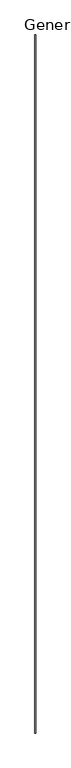
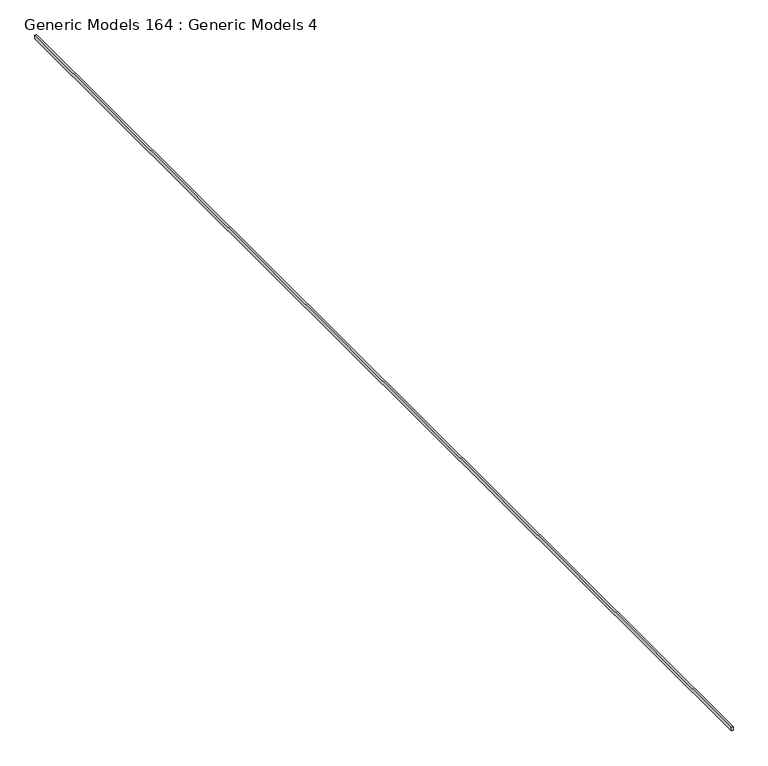
"""IFC4 building model written with IfcOpenShell, lengths in millimetres: proxy geometry, Generic Models 164 : Generic Models 4."""

from ifc_helpers import new_model, si_unit, origin, place, context, project, spatial, faceted_brep, source, transform, mapped, element, save


def generic_models_164_generic_models_4_ca790fd0(model_context):
    return source(origin(), model_context, "Body", "Brep", [
        faceted_brep([(-10252.9339552, -5493.3230338, 122820.8249647), (-10252.9339552, -5493.3230338, 122811.2999647), (-10252.9339552, -5493.3230338, 122784.1984874), (-10236.1097239, -5493.3230338, 122784.1984874), (-10236.1097239, -5493.3230338, 122820.8249647), (-10252.9339552, 7054.2769662, 122820.8249647), (-10236.1097239, 7054.2769662, 122820.8249647), (-10236.1097239, 7054.2769662, 122784.1984874), (-10252.9339552, 7054.2769662, 122784.1984874), (-10252.9339552, 7054.2769662, 122811.2999647)], [[[0, 1, 2, 3, 4]], [[5, 6, 7, 8, 9]], [[2, 1, 0, 5, 9, 8]], [[3, 2, 8, 7]], [[4, 3, 7, 6]], [[0, 4, 6, 5]]]),
    ])


if __name__ == "__main__":
    model = new_model("IFC4")
    model_context = context("Model", 3, world=origin())
    ifc_project = project(units=[si_unit("LENGTHUNIT", "METRE", prefix="MILLI")], contexts=[model_context])
    site = spatial("IfcSite", under=ifc_project)
    building = spatial("IfcBuilding", under=site)
    placement = place(None, origin())
    generic_models_164_generic_models_4_shape = generic_models_164_generic_models_4_ca790fd0(model_context)
    element("IfcBuildingElementProxy", 1, Name="Generic Models 164 : Generic Models 4", ObjectType="Generic Models 164 : Generic Models 4", at=placement, inside=building, context=model_context, shape_type="MappedRepresentation", body=[
        mapped(generic_models_164_generic_models_4_shape, transform((0.0, 0.0, 0.0), x_axis=(1.0, 0.0, 0.0), y_axis=(0.0, 1.0, 0.0), z_axis=(0.0, 0.0, 1.0))),
    ])
    save(model, "model.ifc")

# Revit data of these elements
# Element 1 (IfcBuildingElementProxy, "Generic Models 164 : Generic Models 4")
#   Materials on its faces: "_MORTAR SETTING BED"
# Materials
#   "_MORTAR SETTING BED": class "Generic", colour RGB 191 191 191, transparency 0, Cost = 0
